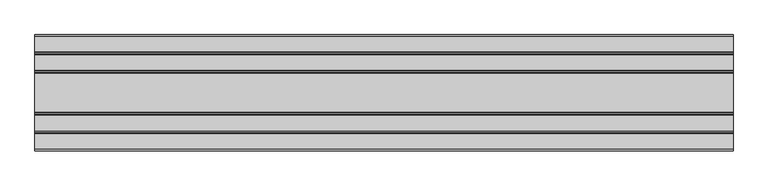
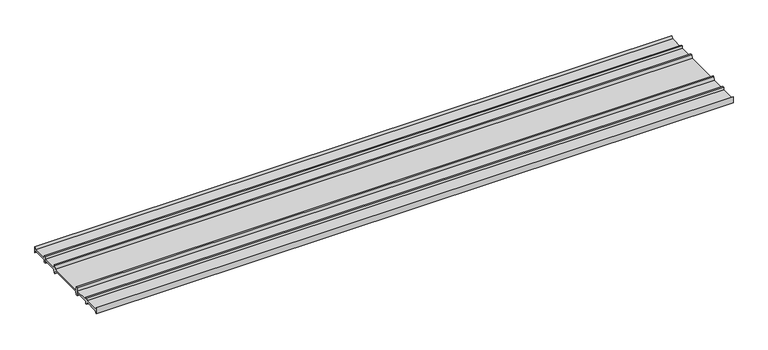
"""IFC4 building model written with IfcOpenShell, lengths in millimetres: proxy geometry, TN_Гидрошпонка ТН Фундамент : Гидрошпонка ТН Фундамент ТШ-В-250."""

from ifc_helpers import new_model, si_unit, frame, origin, place, context, project, spatial, polyline, outline, extrude, source, transform, mapped, element, save


def specialty_equipment_d3ba57ba(model_context):
    return source(origin(), model_context, "Body", "SweptSolid", [
        extrude(outline(polyline([(-83.280218, -5.7544352), (-86.719782, -5.7544352), (-87.7344441, 0.0), (-121.5809483, 0.0), (-125.0, -5.5044352), (-125.0, 9.4955648), (-121.5809483, 3.9911296), (-87.7344441, 3.9911296), (-86.719782, 9.7455648), (-83.280218, 9.7455648), (-82.2655559, 3.9911296), (-48.0288318, 3.9911296), (-46.7513068, 11.75), (-43.2486932, 11.75), (-41.9722041, 3.9974211), (41.9722041, 3.9974211), (43.2486932, 11.75), (46.7513068, 11.75), (48.0288318, 3.9911296), (82.2655559, 3.9911296), (83.280218, 9.7455648), (86.719782, 9.7455648), (87.7344441, 3.9911296), (121.5809483, 3.9911296), (125.0, 9.4955648), (125.0, -5.5044352), (121.5809483, 0.0), (87.7344441, 0.0), (86.719782, -5.7544352), (83.280218, -5.7544352), (82.2655559, 0.0), (48.1139579, 0.0), (46.7513068, -8.2758715), (43.2486932, -8.2758715), (41.8860421, 0.0), (-41.8860421, 0.0), (-43.2486932, -8.2758715), (-46.7513068, -8.2758715), (-48.1139579, 0.0), (-82.2655559, 0.0), (-83.280218, -5.7544352)])), frame((0.0, 0.0, 0.0), z_axis=(1.0, 0.0, 0.0), x_axis=(0.0, 1.0, 0.0)), (0.0, 0.0, 1.0), 1500.0),
    ])


if __name__ == "__main__":
    model = new_model("IFC4")
    model_context = context("Model", 3, world=origin())
    ifc_project = project(units=[si_unit("LENGTHUNIT", "METRE", prefix="MILLI")], contexts=[model_context])
    site = spatial("IfcSite", under=ifc_project)
    building = spatial("IfcBuilding", under=site)
    placement = place(None, origin())
    specialty_equipment_shape = specialty_equipment_d3ba57ba(model_context)
    element("IfcBuildingElementProxy", 1, Name="TN_Гидрошпонка ТН Фундамент : Гидрошпонка ТН Фундамент ТШ-В-250", ObjectType="TN_Гидрошпонка ТН Фундамент : Гидрошпонка ТН Фундамент ТШ-В-250", at=placement, inside=building, context=model_context, shape_type="MappedRepresentation", body=[
        mapped(specialty_equipment_shape, transform((0.0, 0.0, 0.0), x_axis=(1.0, 0.0, 0.0), y_axis=(0.0, 1.0, 0.0), z_axis=(0.0, 0.0, 1.0))),
    ])
    save(model, "model.ifc")

# Revit data of these elements
# Type "TN_Гидрошпонка ТН Фундамент : Гидрошпонка ТН Фундамент ТШ-В-250"
#   Description = "Внутренние гидроизоляционные шпонки ТН Фундамент ТШ-В предназначены для герметизации технологических швов бетонирования при строительстве подземных и заглубленных конструкций зданий и сооружений различного назначения и класса ответственности."
#   Type Comments = "п.м."
#   Manufacturer = "ТехноНИКОЛЬ"
#   URL = "https://nav.tn.ru/catalog/gidroizolyatsiya/komplektatsiya-dlya-gidroizolyatsii/gidroshponki-tekhnonikol-fundament-tsh-v/"
#   ADSK_Примечание = ""
#   ADSK_Обозначение [instance default] = "ТехноНИКОЛЬ"
#   ADSK_Наименование = "Гидрошпонка ТН Фундамент ТШ-В-250"
#   ADSK_Масса_Текст = ""
#   ADSK_Марка = ""
#   ADSK_Код изделия = "66675"
#   ADSK_Завод-изготовитель [instance default] = "ТехноНИКОЛЬ"
#   ADSK_Единица измерения [instance default] = "п.м."
#   ADSK_Группирование = "Гидрошпонки"
#   ADSK_URL страницы изделия = "https://nav.tn.ru/catalog/gidroizolyatsiya/komplektatsiya-dlya-gidroizolyatsii/gidroshponki-tekhnonikol-fundament-tsh-v/"
#   ADSK_URL документации изделия = "https://nav.tn.ru/upload/iblock/a6b/ewrhpb0y1xrl8jlgtx64kildvudhcq55/Tekhlist-7.401_Gidroshponki-TN-Fundament-TSH_V_RU_ru.pdf"
#   built-in parameter 1001306 [instance default] = 3.28084 (stored number, unit not read)
#   ADSK_Размер_Длина [instance default] = 1000 mm
#   ADSK_Количество [instance default] = 1
#   Гидрошпонка ТН Фундамент ТШ-Н-210 = no
#   Гидрошпонка ТН Фундамент ДШП-В-50 = no
#   Гидрошпонка ТН Фундамент ДШП-В-20 = no
#   Гидрошпонка ТН Фундамент ДШ-В-280 = no
#   Гидрошпонка ТН Фундамент ДШ-В-250 = no
#   Гидрошпонка ТН Фундамент ТШ-В-250 = yes
#   Гидрошпонка ТН Фундамент ТПС-В 140-1 = no
#   Гидрошпонка ТН Фундамент ДШ-Н-280 = no
#   Гидрошпонка ТН Фундамент ДШ-Н-250 = no
#   Гидрошпонка ТН Фундамент ТПС-В 100-2 = no
#   Гидрошпонка ТН Фундамент ТШ-Н-250 = no
#   Гидрошпонка ТН Фундамент ТШ-В-210 = no
#   Материал = TN_ПВХ_Черный
#   Default Elevation = 0
# Element 1 (IfcBuildingElementProxy, "TN_Гидрошпонка ТН Фундамент : Гидрошпонка ТН Фундамент ТШ-В-250")
#   built-in parameter 1001306 = 4.92126 (stored number, unit not read)
#   ADSK_Размер_Длина = 1500 mm
#   ADSK_Количество = 1.5
#   Materials on its faces: "TN_ПВХ_Черный"
# Materials
#   "TN_ПВХ_Черный": class "Типовые", colour RGB 48 48 48, transparency 0, Cost = 0
